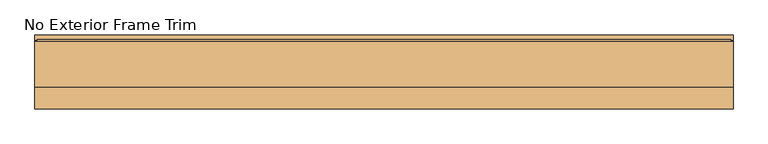
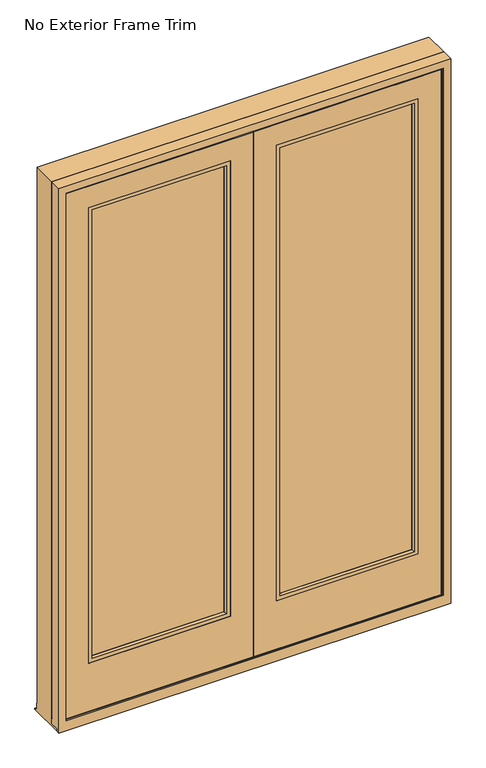
"""IFC4 building model written with IfcOpenShell, lengths in millimetres: door geometry, Door-In_Swing-Milgard-Essence-2_Panel : No Exterior Frame Trim."""

import ifcopenshell
import ifcopenshell.guid

model = None  # the IFC model being written
_history = None  # IfcOwnerHistory: only IFC2X3 demands one
_inside = {}  # id of a spatial element -> (the spatial element, [elements in it])
_under = {}  # id of a project, library or spatial element -> (it, [spatial elements below it])
_declared = {}  # id of a project -> (the project, [libraries it declares])
_typed = {}  # id of a type object -> (the type object, [elements of that type])
_made_of = {}  # id of a material, layer set ... -> (it, [elements and type objects made of it])


def new_model(schema):
    """Start an empty IFC model of exactly this schema.

    Asked for "IFC4X3", IfcOpenShell would pick the latest addendum, in which some entities
    have other attributes; the version numbers below select the first issue.
    IFC2X3 requires an IfcOwnerHistory on every rooted entity: one is made here for all.
    """
    global model, _history
    if schema == "IFC4X3":
        model = ifcopenshell.file(schema_version=(4, 3, 0, 0))
    else:
        model = ifcopenshell.file(schema=schema)
    _inside.clear()
    _under.clear()
    _declared.clear()
    _typed.clear()
    _made_of.clear()
    _history = None
    if model.schema == "IFC2X3":
        org = make("IfcOrganization", Name="unknown")
        user = make(
            "IfcPersonAndOrganization",
            ThePerson=make("IfcPerson", FamilyName="unknown"),
            TheOrganization=org,
        )
        app = make(
            "IfcApplication",
            ApplicationDeveloper=org,
            Version="unknown",
            ApplicationFullName="unknown",
            ApplicationIdentifier="unknown",
        )
        _history = make(
            "IfcOwnerHistory",
            OwningUser=user,
            OwningApplication=app,
            ChangeAction="ADDED",
            CreationDate=0,
        )
    return model


def make(cls, **values):
    """One entity of the class cls with the attributes given. An attribute that is None is left unset."""
    return model.create_entity(
        cls, **{name: value for name, value in values.items() if value is not None}
    )


def rooted(cls, **values):
    """An entity with a GlobalId (a new one), such as an element, a storey or a relation."""
    return make(cls, GlobalId=ifcopenshell.guid.new(), OwnerHistory=_history, **values)


def si_unit(unit_type, name, prefix=None):
    """IfcSIUnit, for example si_unit("LENGTHUNIT", "METRE", prefix="MILLI")."""
    return make("IfcSIUnit", UnitType=unit_type, Prefix=prefix, Name=name)


def assignment(units):
    """IfcUnitAssignment: the units of a project."""
    return None if units is None else make("IfcUnitAssignment", Units=units)


def point(xyz):
    """IfcCartesianPoint."""
    return None if xyz is None else make("IfcCartesianPoint", Coordinates=xyz)


def direction(xyz):
    """IfcDirection."""
    return None if xyz is None else make("IfcDirection", DirectionRatios=xyz)


def frame(location, z_axis=None, x_axis=None):
    """IfcAxis2Placement3D, a coordinate frame: its origin and axes. An axis left out is left unset."""
    return make(
        "IfcAxis2Placement3D",
        Location=point(location),
        Axis=direction(z_axis),
        RefDirection=direction(x_axis),
    )


def origin():
    """The frame at (0, 0, 0) with its axes left unset."""
    return frame((0.0, 0.0, 0.0))


def place(relative_to, where):
    """IfcLocalPlacement: puts the frame where relative to a parent placement (None: the world)."""
    return make(
        "IfcLocalPlacement", PlacementRelTo=relative_to, RelativePlacement=where
    )


def context(
    kind, dimensions, precision=None, world=None, true_north=None, identifier=None
):
    """IfcGeometricRepresentationContext, for example the 3D "Model" context."""
    return make(
        "IfcGeometricRepresentationContext",
        ContextIdentifier=identifier,
        ContextType=kind,
        CoordinateSpaceDimension=dimensions,
        Precision=precision,
        WorldCoordinateSystem=world,
        TrueNorth=true_north,
    )


def project(units=None, contexts=None):
    """IfcProject with its units and contexts."""
    return rooted(
        "IfcProject",
        Name="project",
        RepresentationContexts=contexts,
        UnitsInContext=assignment(units),
    )


def spatial(cls, under=None, at=None, **own):
    """A site, building, storey or space (cls), placed at a placement, below another one or the project."""
    s = rooted(cls, ObjectPlacement=at, **own)
    if under is not None:
        _under.setdefault(under.id(), (under, []))[1].append(s)
    return s


def polyline(points):
    """IfcPolyline through the points."""
    return make("IfcPolyline", Points=[point(p) for p in points])


def outline(outer, holes=None, kind="AREA"):
    """IfcArbitraryClosedProfileDef: a profile drawn as a closed curve; with holes, ...WithVoids."""
    if holes is None:
        return make("IfcArbitraryClosedProfileDef", ProfileType=kind, OuterCurve=outer)
    return make(
        "IfcArbitraryProfileDefWithVoids",
        ProfileType=kind,
        OuterCurve=outer,
        InnerCurves=holes,
    )


def extrude(swept, where, along, depth):
    """IfcExtrudedAreaSolid: the profile swept, set in the frame where, extruded along a direction by depth."""
    return make(
        "IfcExtrudedAreaSolid",
        SweptArea=swept,
        Position=where,
        ExtrudedDirection=direction(along),
        Depth=depth,
    )


def faces_of(points, faces, orient=None, outer=None):
    """IfcFace entities. A face is a list of loops; a loop is a list of indices into points, from 0.

    orient and outer hold one flag for each loop. By default every Orientation is true, the
    first loop of a face is its IfcFaceOuterBound and the others are IfcFaceBound.
    """
    made = []
    for i, loops in enumerate(faces):
        bounds = []
        for j, loop in enumerate(loops):
            is_outer = j == 0 if outer is None else outer[i][j]
            bounds.append(
                make(
                    "IfcFaceOuterBound" if is_outer else "IfcFaceBound",
                    Bound=make("IfcPolyLoop", Polygon=[points[k] for k in loop]),
                    Orientation=True if orient is None else orient[i][j],
                )
            )
        made.append(make("IfcFace", Bounds=bounds))
    return made


def faceted_brep(points, faces, orient=None, outer=None, voids=None):
    """IfcFacetedBrep: a solid bounded by flat faces; with voids (closed shells), ...WithVoids."""
    shared = [point(p) for p in points]
    hull = make("IfcClosedShell", CfsFaces=faces_of(shared, faces, orient, outer))
    if voids is None:
        return make("IfcFacetedBrep", Outer=hull)
    return make(
        "IfcFacetedBrepWithVoids",
        Outer=hull,
        Voids=[
            make(cls, CfsFaces=faces_of(shared, fs, o, b)) for cls, fs, o, b in voids
        ],
    )


def shape(context_of_items, identifier, shape_type, items):
    """IfcShapeRepresentation: the items that make up one representation, for example the "Body"."""
    return make(
        "IfcShapeRepresentation",
        ContextOfItems=context_of_items,
        RepresentationIdentifier=identifier,
        RepresentationType=shape_type,
        Items=items,
    )


def source(mapping_origin, context_of_items, identifier, shape_type, items):
    """IfcRepresentationMap: a shape defined once, which mapped items show again and again."""
    return make(
        "IfcRepresentationMap",
        MappingOrigin=mapping_origin,
        MappedRepresentation=shape(context_of_items, identifier, shape_type, items),
    )


def transform(
    local_origin,
    x_axis=None,
    y_axis=None,
    z_axis=None,
    scale=None,
    scale2=None,
    scale3=None,
    uniform=True,
):
    """IfcCartesianTransformationOperator3D, or its non-uniform kind. x_axis, y_axis, z_axis: its Axis1, 2, 3."""
    if uniform:
        return make(
            "IfcCartesianTransformationOperator3D",
            Axis1=direction(x_axis),
            Axis2=direction(y_axis),
            LocalOrigin=point(local_origin),
            Scale=scale,
            Axis3=direction(z_axis),
        )
    return make(
        "IfcCartesianTransformationOperator3DnonUniform",
        Axis1=direction(x_axis),
        Axis2=direction(y_axis),
        LocalOrigin=point(local_origin),
        Scale=scale,
        Axis3=direction(z_axis),
        Scale2=scale2,
        Scale3=scale3,
    )


def mapped(mapping_source, mapping_target):
    """IfcMappedItem: shows the shape of a source again, moved by a transform."""
    return make(
        "IfcMappedItem", MappingSource=mapping_source, MappingTarget=mapping_target
    )


def made_of(thing, what):
    """Note that an element or type object is made of a material, layer set ...; save() writes the relation."""
    if what is not None:
        _made_of.setdefault(what.id(), (what, []))[1].append(thing)
    return thing


def element(
    cls,
    number,
    at=None,
    inside=None,
    cuts=None,
    type_object=None,
    material=None,
    context=None,
    identifier="Body",
    shape_type=None,
    held_by="IfcProductDefinitionShape",
    body=None,
    shapes=None,
    **own,
):
    """One element of the class cls, such as IfcWall. Its Tag is "e" and its number.

    at: its placement. inside: the storey or other place that contains it. cuts: it is an
    opening in that element (IfcRelVoidsElement). A single representation is given by context,
    identifier, shape_type and body (its items); several are given by shapes. held_by: the class
    of the entity that holds the representations. save() writes the other relations.
    """
    e = rooted(cls, Tag="e%d" % number, ObjectPlacement=at, **own)
    if body is not None:
        shapes = [shape(context, identifier, shape_type, body)]
    if shapes is not None:
        e.Representation = make(held_by, Representations=shapes)
    if inside is not None:
        _inside.setdefault(inside.id(), (inside, []))[1].append(e)
    if cuts is not None:
        rooted(
            "IfcRelVoidsElement", RelatingBuildingElement=cuts, RelatedOpeningElement=e
        )
    if type_object is not None:
        _typed.setdefault(type_object.id(), (type_object, []))[1].append(e)
    return made_of(e, material)


def aggregate(whole, parts):
    """IfcRelAggregates: a whole, such as a stair, and the parts it consists of."""
    return rooted("IfcRelAggregates", RelatingObject=whole, RelatedObjects=parts)


def save(model, path):
    """Write the relations noted so far, then the file.

    IfcRelAggregates (storeys below a building ...), IfcRelContainedInSpatialStructure (elements
    in a storey), IfcRelDefinesByType, IfcRelAssociatesMaterial and IfcRelDeclares: one each for
    every whole, place, type object, material and project.
    """
    for whole, parts in _under.values():
        aggregate(whole, parts)
    for where, things in _inside.values():
        rooted(
            "IfcRelContainedInSpatialStructure",
            RelatedElements=things,
            RelatingStructure=where,
        )
    for kind, things in _typed.values():
        rooted("IfcRelDefinesByType", RelatedObjects=things, RelatingType=kind)
    for what, things in _made_of.values():
        rooted("IfcRelAssociatesMaterial", RelatedObjects=things, RelatingMaterial=what)
    for by, libraries in _declared.values():
        rooted("IfcRelDeclares", RelatingContext=by, RelatedDefinitions=libraries)
    model.write(path)


def no_exterior_frame_trim_3783c24b(model_context):
    return source(origin(), model_context, "Body", "SolidModel", [
        extrude(outline(polyline([(591.4684989, -28.575), (591.4684989, -53.975), (54.2422052, -53.975), (54.2422052, -28.575), (591.4684989, -28.575)])), frame((0.0, 0.0, 245.0465023), z_axis=(0.0, 0.0, 1.0), x_axis=(1.0, 0.0, 0.0)), (0.0, 0.0, 1.0), 1856.965426),
        faceted_brep([(-22.501829, -56.3244996, 39.0524923), (-20.0336081, -53.2765006, 39.0524923), (47.7525111, -53.2765006, 39.0524923), (47.7525111, -55.0418002, 39.0524923), (61.9460004, -55.0418002, 39.0524923), (63.4695489, -53.975, 39.0524923), (66.9526032, -53.975, 39.0524923), (66.9526032, -55.857139, 39.0524923), (66.6827722, -56.3244996, 39.0524923), (579.0279319, -56.3244996, 39.0524923), (578.7581009, -55.857139, 39.0524923), (578.7581009, -53.975, 39.0524923), (582.2411552, -53.975, 39.0524923), (583.7647037, -55.0418002, 39.0524923), (597.9581931, -55.0418002, 39.0524923), (597.9581931, -53.2765006, 39.0524923), (665.7443122, -53.2765006, 39.0524923), (668.2125331, -56.3244996, 39.0524923), (685.524688, -56.3244996, 39.0524923), (685.524688, -64.6430002, 39.0524923), (-39.8139839, -64.6430002, 39.0524923), (-39.8139839, -56.3244996, 39.0524923), (-22.501829, -56.3244996, 56.3603664), (-20.0336081, -53.2765006, 58.8285873), (-22.501829, -56.3244996, 2178.7559624), (-20.0336081, -53.2765006, 2176.2877415), (-20.0336081, -53.2765006, 238.4932696), (-21.4631194, -55.0418002, 238.4932696), (-21.4631194, -55.0418002, 252.686759), (-20.5992417, -53.975, 254.2103075), (-20.5992417, -53.975, 257.6933617), (-22.1233678, -55.857139, 257.6933617), (-22.501829, -56.3244996, 257.4235308), (-39.8139839, -53.2765006, 58.8285873), (-39.8139839, -53.2765006, 238.4932696), (665.7443122, -53.2765006, 2176.2877415), (665.7443122, -53.2765006, 238.4932696), (685.524688, -53.2765006, 238.4932696), (685.524688, -53.2765006, 58.8285873), (665.7443122, -53.2765006, 58.8285873), (597.9581931, -53.2765006, 58.8285873), (47.7525111, -53.2765006, 58.8285873), (47.7525111, -53.2765006, 2108.5016224), (47.7525111, -53.2765006, 238.4932696), (597.9581931, -53.2765006, 238.4932696), (597.9581931, -53.2765006, 2108.5016224), (47.7525111, -55.0418002, 57.3990759), (47.7525111, -55.0418002, 2108.5016224), (47.7525111, -55.0418002, 257.6933617), (47.7525111, -53.975, 257.6933617), (47.7525111, -53.975, 254.2103075), (47.7525111, -55.0418002, 252.686759), (47.7525111, -55.0418002, 238.4932696), (61.9460004, -55.0418002, 57.3990759), (583.7647037, -55.0418002, 57.3990759), (597.9581931, -55.0418002, 57.3990759), (61.9460004, -55.0418002, 252.686759), (61.9460004, -55.0418002, 238.4932696), (597.9581931, -55.0418002, 2108.5016224), (597.9581931, -55.0418002, 257.6933617), (583.7647037, -55.0418002, 257.6933617), (583.7647037, -55.0418002, 2094.3081331), (61.9460004, -55.0418002, 2094.3081331), (61.9460004, -55.0418002, 257.6933617), (597.9581931, -55.0418002, 252.686759), (597.9581931, -55.0418002, 238.4932696), (583.7647037, -55.0418002, 238.4932696), (583.7647037, -55.0418002, 252.686759), (63.4695489, -53.975, 58.2629537), (63.4695489, -53.975, 254.2103075), (63.4695489, -53.975, 238.4932696), (63.4695489, -53.975, 2092.7845845), (63.4695489, -53.975, 257.6933617), (66.9526032, -53.975, 58.2629537), (578.7581009, -53.975, 58.2629537), (582.2411552, -53.975, 58.2629537), (582.2411552, -53.975, 2092.7845845), (582.2411552, -53.975, 257.6933617), (597.9581931, -53.975, 257.6933617), (597.9581931, -53.975, 254.2103075), (582.2411552, -53.975, 254.2103075), (582.2411552, -53.975, 238.4932696), (578.7581009, -53.975, 238.4932696), (578.7581009, -53.975, 254.2103075), (66.9526032, -53.975, 254.2103075), (66.9526032, -53.975, 238.4932696), (66.9526032, -53.975, 2089.3015303), (66.9526032, -53.975, 257.6933617), (578.7581009, -53.975, 257.6933617), (578.7581009, -53.975, 2089.3015303), (-39.8139839, -53.975, 254.2103075), (-39.8139839, -53.975, 257.6933617), (685.524688, -53.975, 257.6933617), (685.524688, -53.975, 254.2103075), (666.3099458, -53.975, 254.2103075), (666.3099458, -53.975, 257.6933617), (66.9526032, -55.857139, 56.7388275), (66.9526032, -55.0418002, 252.686759), (66.9526032, -55.0418002, 238.4932696), (66.9526032, -55.857139, 2089.3015303), (66.9526032, -55.857139, 257.6933617), (66.6827722, -56.3244996, 56.3603664), (62.3383529, -63.8492502, 2093.9157805), (62.3383529, -63.8492502, 253.0791115), (597.9581931, -63.8492502, 2108.5016224), (47.7525111, -63.8492502, 2108.5016224), (47.7525111, -63.8492502, 238.4932696), (597.9581931, -63.8492502, 238.4932696), (583.3723512, -63.8492502, 2093.9157805), (583.3723512, -63.8492502, 253.0791115), (47.7525111, -64.6430002, 2108.5016224), (47.7525111, -64.6430002, 238.4932696), (685.524688, -64.6430002, 2196.0681173), (-39.8139839, -64.6430002, 2196.0681173), (597.9581931, -64.6430002, 2108.5016224), (597.9581931, -64.6430002, 238.4932696), (-39.8139839, -56.3244996, 2196.0681173), (-39.8139839, -56.3244996, 257.4235308), (-39.8139839, -55.857139, 257.6933617), (-39.8139839, -55.0418002, 252.686759), (-39.8139839, -55.0418002, 238.4932696), (-39.8139839, -56.3244996, 56.3603664), (668.2125331, -56.3244996, 56.3603664), (685.524688, -56.3244996, 56.3603664), (685.524688, -56.3244996, 2196.0681173), (685.524688, -56.3244996, 257.4235308), (668.2125331, -56.3244996, 257.4235308), (668.2125331, -56.3244996, 2178.7559624), (578.7581009, -55.857139, 2089.3015303), (667.8340719, -55.857139, 257.6933617), (667.1738236, -55.0418002, 252.686759), (667.1738236, -55.0418002, 238.4932696), (578.7581009, -55.857139, 56.7388275), (578.7581009, -55.857139, 257.6933617), (578.7581009, -55.0418002, 238.4932696), (578.7581009, -55.0418002, 252.686759), (579.0279319, -56.3244996, 56.3603664), (685.524688, -55.0418002, 238.4932696), (685.524688, -55.0418002, 252.686759), (685.524688, -55.857139, 257.6933617)], [[[0, 1, 2, 3, 4, 5, 6, 7, 8, 9, 10, 11, 12, 13, 14, 15, 16, 17, 18, 19, 20, 21]], [[1, 0, 22, 23]], [[24, 25, 26, 27, 28, 29, 30, 31, 32]], [[2, 1, 23, 33, 34, 26, 25, 35, 36, 37, 38, 39, 16, 15, 40, 41], [42, 43, 44, 45]], [[3, 2, 41, 46]], [[42, 47, 48, 49, 50, 51, 52, 43]], [[4, 3, 46, 53]], [[14, 13, 54, 55]], [[52, 51, 56, 57]], [[47, 58, 59, 60, 61, 62, 63, 48]], [[64, 65, 66, 67]], [[5, 4, 53, 68]], [[57, 56, 69, 70]], [[62, 71, 72, 63]], [[6, 5, 68, 73]], [[12, 11, 74, 75]], [[71, 76, 77, 78, 79, 80, 81, 82, 83, 84, 85, 70, 69, 50, 49, 72], [86, 87, 88, 89]], [[90, 91, 30, 29]], [[92, 93, 94, 95]], [[7, 6, 73, 96]], [[85, 84, 97, 98]], [[86, 99, 100, 87]], [[8, 7, 96, 101]], [[99, 102, 103, 100]], [[104, 105, 106, 107], [102, 108, 109, 103]], [[106, 105, 110, 111]], [[20, 19, 112, 113], [114, 115, 111, 110]], [[21, 20, 113, 116, 117, 118, 91, 90, 119, 120, 34, 33, 121]], [[18, 17, 122, 123]], [[0, 21, 121, 22]], [[116, 124, 125, 126, 127, 24, 32, 117]], [[25, 24, 127, 35]], [[42, 45, 58, 47]], [[62, 61, 76, 71]], [[86, 89, 128, 99]], [[102, 99, 128, 108]], [[105, 104, 114, 110]], [[113, 112, 124, 116]], [[17, 16, 39, 122]], [[35, 127, 126, 129, 95, 94, 130, 131, 36]], [[15, 14, 55, 40]], [[58, 45, 44, 65, 64, 79, 78, 59]], [[13, 12, 75, 54]], [[81, 80, 67, 66]], [[76, 61, 60, 77]], [[11, 10, 132, 74]], [[128, 89, 88, 133]], [[83, 82, 134, 135]], [[10, 9, 136, 132]], [[108, 128, 133, 109]], [[114, 104, 107, 115]], [[124, 112, 19, 18, 123, 38, 37, 137, 138, 93, 92, 139, 125]], [[107, 106, 111, 115]], [[118, 117, 32, 31]], [[125, 139, 129, 126]], [[103, 109, 133, 100]], [[78, 77, 60, 59]], [[72, 49, 48, 63]], [[88, 87, 100, 133]], [[91, 118, 31, 30]], [[139, 92, 95, 129]], [[119, 90, 29, 28]], [[93, 138, 130, 94]], [[80, 79, 64, 67]], [[84, 83, 135, 97]], [[50, 69, 56, 51]], [[120, 119, 28, 27]], [[138, 137, 131, 130]], [[97, 135, 134, 98]], [[44, 43, 52, 57, 70, 85, 98, 134, 82, 81, 66, 65]], [[34, 120, 27, 26]], [[137, 37, 36, 131]], [[121, 33, 23, 22]], [[38, 123, 122, 39]], [[41, 40, 55, 54, 75, 74, 132, 136, 101, 96, 73, 68, 53, 46]], [[9, 8, 101, 136]]]),
        faceted_brep([(-39.8139839, -20.1929984, 39.0524923), (-39.8139839, -56.3244996, 39.0524923), (-39.8139839, -56.3244996, 2196.0681173), (-39.8139839, -20.1929984, 2196.0681173), (685.524688, -56.3244996, 39.0524923), (685.524688, -20.1929984, 39.0524923), (685.524688, -20.1929984, 2196.0681173), (685.524688, -56.3244996, 2196.0681173), (66.7863819, -27.3270033, 257.5271404), (578.9243222, -27.3270033, 257.5271404), (586.0583272, -20.1929984, 250.3931355), (59.6523769, -20.1929984, 250.3931355), (586.0583272, -20.1929984, 2096.6017565), (59.6523769, -20.1929984, 2096.6017565), (669.6356705, -56.3244996, 55.4786786), (-23.9249664, -56.3244996, 55.4786786), (-23.9249664, -56.3244996, 2180.1790999), (669.6356705, -56.3244996, 2180.1790999), (666.5876715, -53.2765006, 57.9468995), (-20.8769674, -53.2765006, 57.9468995), (666.5876715, -53.2765006, 2177.1311009), (-20.8769674, -53.2765006, 2177.1311009), (594.7531877, -53.2765006, 241.698275), (50.9575164, -53.2765006, 241.698275), (50.9575164, -53.2765006, 2105.296617), (594.7531877, -53.2765006, 2105.296617), (594.7531877, -50.8481081, 241.698275), (50.9575164, -50.8481081, 241.698275), (49.0643221, -50.8481081, 2107.1898114), (596.646382, -50.8481081, 2107.1898114), (596.646382, -50.8481081, 239.8050807), (49.0643221, -50.8481081, 239.8050807), (594.7531877, -50.8481081, 2105.296617), (50.9575164, -50.8481081, 2105.296617), (597.9581931, -46.8107689, 238.4932696), (47.7525111, -46.8107689, 238.4932696), (597.9581931, -27.8384005, 238.4932696), (581.6983611, -27.8384005, 238.4932696), (580.9617616, -28.575, 238.4932696), (578.9243222, -28.575, 238.4932696), (578.9243222, -27.8384005, 238.4932696), (66.7863819, -27.8384005, 238.4932696), (66.7863819, -28.575, 238.4932696), (64.7489425, -28.575, 238.4932696), (64.012343, -27.8384005, 238.4932696), (47.7525111, -27.8384005, 238.4932696), (597.9581931, -27.8384005, 254.7531016), (581.6983611, -27.8384005, 254.7531016), (578.9243222, -27.8384005, 254.7531016), (66.7863819, -27.8384005, 254.7531016), (64.012343, -27.8384005, 254.7531016), (47.7525111, -27.8384005, 254.7531016), (64.7489425, -28.575, 255.4897011), (47.7525111, -28.575, 255.4897011), (578.9243222, -28.575, 255.4897011), (66.7863819, -28.575, 255.4897011), (597.9581931, -28.575, 255.4897011), (580.9617616, -28.575, 255.4897011), (597.9581931, -28.575, 257.5271404), (580.9617616, -28.575, 257.5271404), (580.9617616, -28.575, 2091.505191), (64.7489425, -28.575, 2091.505191), (64.7489425, -28.575, 257.5271404), (47.7525111, -28.575, 257.5271404), (578.9243222, -28.575, 257.5271404), (66.7863819, -28.575, 257.5271404), (66.7863819, -28.575, 2089.4677516), (578.9243222, -28.575, 2089.4677516), (597.9581931, -27.8384005, 257.5271404), (581.6983611, -27.8384005, 257.5271404), (64.012343, -27.8384005, 257.5271404), (47.7525111, -27.8384005, 257.5271404), (66.7863819, -27.3270033, 2089.4677516), (64.012343, -27.8384005, 2092.2417904), (581.6983611, -27.8384005, 2092.2417904), (597.9581931, -27.8384005, 2108.5016224), (47.7525111, -27.8384005, 2108.5016224), (47.7525111, -46.8107689, 2108.5016224), (578.9243222, -27.3270033, 2089.4677516), (597.9581931, -46.8107689, 2108.5016224)], [[[0, 1, 2, 3]], [[4, 5, 6, 7]], [[8, 9, 10, 11]], [[0, 3, 6, 5], [11, 10, 12, 13]], [[4, 1, 0, 5]], [[2, 1, 4, 7], [14, 15, 16, 17]], [[15, 14, 18, 19]], [[20, 21, 19, 18], [22, 23, 24, 25]], [[23, 22, 26, 27]], [[28, 29, 30, 31], [27, 26, 32, 33]], [[31, 30, 34, 35]], [[35, 34, 36, 37, 38, 39, 40, 41, 42, 43, 44, 45]], [[37, 36, 46, 47]], [[41, 40, 48, 49]], [[45, 44, 50, 51]], [[51, 50, 52, 53]], [[49, 48, 54, 55]], [[47, 46, 56, 57]], [[53, 52, 43, 42, 55, 54, 39, 38, 57, 56, 58, 59, 60, 61, 62, 63], [64, 65, 66, 67]], [[9, 8, 65, 64]], [[59, 58, 68, 69]], [[63, 62, 70, 71]], [[13, 72, 8, 11]], [[55, 42, 41, 49]], [[72, 66, 65, 8]], [[43, 52, 50, 44]], [[61, 73, 70, 62]], [[73, 74, 69, 68, 75, 76, 71, 70]], [[76, 77, 35, 45, 51, 53, 63, 71]], [[77, 28, 31, 35]], [[33, 24, 23, 27]], [[19, 21, 16, 15]], [[13, 12, 78, 72]], [[66, 72, 78, 67]], [[61, 60, 74, 73]], [[76, 75, 79, 77]], [[28, 77, 79, 29]], [[33, 32, 25, 24]], [[21, 20, 17, 16]], [[6, 3, 2, 7]], [[78, 12, 10, 9]], [[39, 54, 48, 40]], [[67, 78, 9, 64]], [[74, 60, 59, 69]], [[57, 38, 37, 47]], [[79, 75, 68, 58, 56, 46, 36, 34]], [[30, 29, 79, 34]], [[25, 32, 26, 22]], [[17, 20, 18, 14]]]),
        extrude(outline(polyline([(-675.754549, -28.575), (-138.5282552, -28.575), (-138.5282552, -53.975), (-675.754549, -53.975), (-675.754549, -28.575)])), frame((0.0, 0.0, 245.0465023), z_axis=(0.0, 0.0, 1.0), x_axis=(1.0, 0.0, 0.0)), (0.0, 0.0, 1.0), 1856.965426),
        faceted_brep([(-61.784221, -56.3244996, 39.0524923), (-44.4720661, -56.3244996, 39.0524923), (-44.4720661, -64.6430002, 39.0524923), (-769.810738, -64.6430002, 39.0524923), (-769.810738, -56.3244996, 39.0524923), (-752.4985831, -56.3244996, 39.0524923), (-750.0303622, -53.2765006, 39.0524923), (-682.2442431, -53.2765006, 39.0524923), (-682.2442431, -55.0418002, 39.0524923), (-668.0507537, -55.0418002, 39.0524923), (-666.5272052, -53.975, 39.0524923), (-663.044151, -53.975, 39.0524923), (-663.044151, -55.857139, 39.0524923), (-663.3139819, -56.3244996, 39.0524923), (-150.9688223, -56.3244996, 39.0524923), (-151.2386532, -55.857139, 39.0524923), (-151.2386532, -53.975, 39.0524923), (-147.755599, -53.975, 39.0524923), (-146.2320504, -55.0418002, 39.0524923), (-132.0385611, -55.0418002, 39.0524923), (-132.0385611, -53.2765006, 39.0524923), (-64.252442, -53.2765006, 39.0524923), (-61.784221, -56.3244996, 2178.7559624), (-61.784221, -56.3244996, 257.4235308), (-62.1626822, -55.857139, 257.6933617), (-63.6868083, -53.975, 257.6933617), (-63.6868083, -53.975, 254.2103075), (-62.8229306, -55.0418002, 252.686759), (-62.8229306, -55.0418002, 238.4932696), (-64.252442, -53.2765006, 238.4932696), (-64.252442, -53.2765006, 2176.2877415), (-64.252442, -53.2765006, 58.8285873), (-61.784221, -56.3244996, 56.3603664), (-132.0385611, -53.2765006, 58.8285873), (-682.2442431, -53.2765006, 58.8285873), (-750.0303622, -53.2765006, 58.8285873), (-769.810738, -53.2765006, 58.8285873), (-769.810738, -53.2765006, 238.4932696), (-750.0303622, -53.2765006, 238.4932696), (-750.0303622, -53.2765006, 2176.2877415), (-44.4720661, -53.2765006, 238.4932696), (-44.4720661, -53.2765006, 58.8285873), (-132.0385611, -53.2765006, 2108.5016224), (-682.2442431, -53.2765006, 2108.5016224), (-682.2442431, -53.2765006, 238.4932696), (-132.0385611, -53.2765006, 238.4932696), (-132.0385611, -55.0418002, 238.4932696), (-132.0385611, -55.0418002, 252.686759), (-132.0385611, -53.975, 254.2103075), (-132.0385611, -53.975, 257.6933617), (-132.0385611, -55.0418002, 257.6933617), (-132.0385611, -55.0418002, 2108.5016224), (-132.0385611, -55.0418002, 57.3990759), (-146.2320504, -55.0418002, 257.6933617), (-146.2320504, -55.0418002, 2094.3081331), (-668.0507537, -55.0418002, 2094.3081331), (-668.0507537, -55.0418002, 257.6933617), (-682.2442431, -55.0418002, 257.6933617), (-682.2442431, -55.0418002, 2108.5016224), (-682.2442431, -55.0418002, 57.3990759), (-668.0507537, -55.0418002, 57.3990759), (-146.2320504, -55.0418002, 238.4932696), (-146.2320504, -55.0418002, 252.686759), (-682.2442431, -55.0418002, 252.686759), (-668.0507537, -55.0418002, 252.686759), (-668.0507537, -55.0418002, 238.4932696), (-682.2442431, -55.0418002, 238.4932696), (-146.2320504, -55.0418002, 57.3990759), (-147.755599, -53.975, 257.6933617), (-147.755599, -53.975, 2092.7845845), (-147.755599, -53.975, 238.4932696), (-147.755599, -53.975, 254.2103075), (-147.755599, -53.975, 58.2629537), (-151.2386532, -53.975, 238.4932696), (-151.2386532, -53.975, 254.2103075), (-663.044151, -53.975, 254.2103075), (-663.044151, -53.975, 238.4932696), (-666.5272052, -53.975, 238.4932696), (-666.5272052, -53.975, 254.2103075), (-682.2442431, -53.975, 254.2103075), (-682.2442431, -53.975, 257.6933617), (-666.5272052, -53.975, 257.6933617), (-666.5272052, -53.975, 2092.7845845), (-151.2386532, -53.975, 2089.3015303), (-663.044151, -53.975, 2089.3015303), (-663.044151, -53.975, 257.6933617), (-151.2386532, -53.975, 257.6933617), (-666.5272052, -53.975, 58.2629537), (-663.044151, -53.975, 58.2629537), (-769.810738, -53.975, 257.6933617), (-750.5959958, -53.975, 257.6933617), (-750.5959958, -53.975, 254.2103075), (-769.810738, -53.975, 254.2103075), (-151.2386532, -53.975, 58.2629537), (-44.4720661, -53.975, 254.2103075), (-44.4720661, -53.975, 257.6933617), (-151.2386532, -55.857139, 257.6933617), (-151.2386532, -55.857139, 2089.3015303), (-151.2386532, -55.0418002, 238.4932696), (-151.2386532, -55.0418002, 252.686759), (-151.2386532, -55.857139, 56.7388275), (-146.624403, -63.8492502, 253.0791115), (-146.624403, -63.8492502, 2093.9157805), (-150.9688223, -56.3244996, 56.3603664), (-682.2442431, -63.8492502, 2108.5016224), (-682.2442431, -63.8492502, 238.4932696), (-132.0385611, -63.8492502, 238.4932696), (-132.0385611, -63.8492502, 2108.5016224), (-667.6584012, -63.8492502, 253.0791115), (-667.6584012, -63.8492502, 2093.9157805), (-132.0385611, -64.6430002, 238.4932696), (-132.0385611, -64.6430002, 2108.5016224), (-44.4720661, -64.6430002, 2196.0681173), (-769.810738, -64.6430002, 2196.0681173), (-682.2442431, -64.6430002, 2108.5016224), (-682.2442431, -64.6430002, 238.4932696), (-44.4720661, -56.3244996, 56.3603664), (-44.4720661, -55.0418002, 238.4932696), (-44.4720661, -55.0418002, 252.686759), (-44.4720661, -55.857139, 257.6933617), (-44.4720661, -56.3244996, 257.4235308), (-44.4720661, -56.3244996, 2196.0681173), (-752.4985831, -56.3244996, 2178.7559624), (-752.4985831, -56.3244996, 257.4235308), (-769.810738, -56.3244996, 257.4235308), (-769.810738, -56.3244996, 2196.0681173), (-769.810738, -56.3244996, 56.3603664), (-752.4985831, -56.3244996, 56.3603664), (-663.044151, -55.857139, 2089.3015303), (-751.4598736, -55.0418002, 238.4932696), (-751.4598736, -55.0418002, 252.686759), (-752.120122, -55.857139, 257.6933617), (-663.044151, -55.857139, 56.7388275), (-663.044151, -55.0418002, 252.686759), (-663.044151, -55.0418002, 238.4932696), (-663.044151, -55.857139, 257.6933617), (-663.3139819, -56.3244996, 56.3603664), (-769.810738, -55.857139, 257.6933617), (-769.810738, -55.0418002, 252.686759), (-769.810738, -55.0418002, 238.4932696)], [[[0, 1, 2, 3, 4, 5, 6, 7, 8, 9, 10, 11, 12, 13, 14, 15, 16, 17, 18, 19, 20, 21]], [[22, 23, 24, 25, 26, 27, 28, 29, 30]], [[21, 31, 32, 0]], [[20, 33, 34, 7, 6, 35, 36, 37, 38, 39, 30, 29, 40, 41, 31, 21], [42, 43, 44, 45]], [[42, 45, 46, 47, 48, 49, 50, 51]], [[19, 52, 33, 20]], [[51, 50, 53, 54, 55, 56, 57, 58]], [[8, 59, 60, 9]], [[46, 61, 62, 47]], [[63, 64, 65, 66]], [[18, 67, 52, 19]], [[54, 53, 68, 69]], [[61, 70, 71, 62]], [[17, 72, 67, 18]], [[69, 68, 49, 48, 71, 70, 73, 74, 75, 76, 77, 78, 79, 80, 81, 82], [83, 84, 85, 86]], [[10, 87, 88, 11]], [[89, 90, 91, 92]], [[16, 93, 72, 17]], [[94, 26, 25, 95]], [[83, 86, 96, 97]], [[73, 98, 99, 74]], [[15, 100, 93, 16]], [[97, 96, 101, 102]], [[14, 103, 100, 15]], [[104, 105, 106, 107], [102, 101, 108, 109]], [[106, 110, 111, 107]], [[2, 112, 113, 3], [114, 111, 110, 115]], [[1, 116, 41, 40, 117, 118, 94, 95, 119, 120, 121, 112, 2]], [[0, 32, 116, 1]], [[121, 120, 23, 22, 122, 123, 124, 125]], [[4, 126, 127, 5]], [[30, 39, 122, 22]], [[42, 51, 58, 43]], [[54, 69, 82, 55]], [[83, 97, 128, 84]], [[102, 109, 128, 97]], [[107, 111, 114, 104]], [[112, 121, 125, 113]], [[39, 38, 129, 130, 91, 90, 131, 123, 122]], [[5, 127, 35, 6]], [[58, 57, 80, 79, 63, 66, 44, 43]], [[7, 34, 59, 8]], [[82, 81, 56, 55]], [[9, 60, 87, 10]], [[77, 65, 64, 78]], [[11, 88, 132, 12]], [[75, 133, 134, 76]], [[128, 135, 85, 84]], [[109, 108, 135, 128]], [[12, 132, 136, 13]], [[114, 115, 105, 104]], [[125, 124, 137, 89, 92, 138, 139, 37, 36, 126, 4, 3, 113]], [[105, 115, 110, 106]], [[101, 96, 135, 108]], [[124, 123, 131, 137]], [[119, 24, 23, 120]], [[68, 53, 50, 49]], [[95, 25, 24, 119]], [[80, 57, 56, 81]], [[85, 135, 96, 86]], [[137, 131, 90, 89]], [[48, 47, 62, 71]], [[74, 99, 133, 75]], [[78, 64, 63, 79]], [[92, 91, 130, 138]], [[118, 27, 26, 94]], [[99, 98, 134, 133]], [[138, 130, 129, 139]], [[117, 28, 27, 118]], [[40, 29, 28, 117]], [[44, 66, 65, 77, 76, 134, 98, 73, 70, 61, 46, 45]], [[139, 129, 38, 37]], [[33, 52, 67, 72, 93, 100, 103, 136, 132, 88, 87, 60, 59, 34]], [[116, 32, 31, 41]], [[36, 35, 127, 126]], [[13, 136, 103, 14]]]),
        faceted_brep([(-44.4720661, -20.1929984, 39.0524923), (-44.4720661, -20.1929984, 2196.0681173), (-44.4720661, -56.3244996, 2196.0681173), (-44.4720661, -56.3244996, 39.0524923), (-769.810738, -56.3244996, 39.0524923), (-769.810738, -56.3244996, 2196.0681173), (-769.810738, -20.1929984, 2196.0681173), (-769.810738, -20.1929984, 39.0524923), (-151.0724319, -27.3270033, 257.5271404), (-143.938427, -20.1929984, 250.3931355), (-670.3443772, -20.1929984, 250.3931355), (-663.2103723, -27.3270033, 257.5271404), (-143.938427, -20.1929984, 2096.6017565), (-670.3443772, -20.1929984, 2096.6017565), (-753.9217206, -56.3244996, 55.4786786), (-753.9217206, -56.3244996, 2180.1790999), (-60.3610836, -56.3244996, 2180.1790999), (-60.3610836, -56.3244996, 55.4786786), (-63.4090826, -53.2765006, 57.9468995), (-750.8737216, -53.2765006, 57.9468995), (-750.8737216, -53.2765006, 2177.1311009), (-63.4090826, -53.2765006, 2177.1311009), (-679.0392377, -53.2765006, 241.698275), (-679.0392377, -53.2765006, 2105.296617), (-135.2435664, -53.2765006, 2105.296617), (-135.2435664, -53.2765006, 241.698275), (-135.2435664, -50.8481081, 241.698275), (-679.0392377, -50.8481081, 241.698275), (-133.3503721, -50.8481081, 2107.1898114), (-133.3503721, -50.8481081, 239.8050807), (-680.9324321, -50.8481081, 239.8050807), (-680.9324321, -50.8481081, 2107.1898114), (-135.2435664, -50.8481081, 2105.296617), (-679.0392377, -50.8481081, 2105.296617), (-132.0385611, -46.8107689, 238.4932696), (-682.2442431, -46.8107689, 238.4932696), (-132.0385611, -27.8384005, 238.4932696), (-148.298393, -27.8384005, 238.4932696), (-149.0349925, -28.575, 238.4932696), (-151.0724319, -28.575, 238.4932696), (-151.0724319, -27.8384005, 238.4932696), (-663.2103723, -27.8384005, 238.4932696), (-663.2103723, -28.575, 238.4932696), (-665.2478116, -28.575, 238.4932696), (-665.9844111, -27.8384005, 238.4932696), (-682.2442431, -27.8384005, 238.4932696), (-132.0385611, -27.8384005, 254.7531016), (-148.298393, -27.8384005, 254.7531016), (-151.0724319, -27.8384005, 254.7531016), (-663.2103723, -27.8384005, 254.7531016), (-665.9844111, -27.8384005, 254.7531016), (-682.2442431, -27.8384005, 254.7531016), (-132.0385611, -28.575, 255.4897011), (-149.0349925, -28.575, 255.4897011), (-151.0724319, -28.575, 255.4897011), (-663.2103723, -28.575, 255.4897011), (-665.2478116, -28.575, 255.4897011), (-682.2442431, -28.575, 255.4897011), (-132.0385611, -28.575, 257.5271404), (-149.0349925, -28.575, 257.5271404), (-149.0349925, -28.575, 2091.505191), (-665.2478116, -28.575, 2091.505191), (-665.2478116, -28.575, 257.5271404), (-682.2442431, -28.575, 257.5271404), (-663.2103723, -28.575, 257.5271404), (-663.2103723, -28.575, 2089.4677516), (-151.0724319, -28.575, 2089.4677516), (-151.0724319, -28.575, 257.5271404), (-132.0385611, -27.8384005, 257.5271404), (-148.298393, -27.8384005, 257.5271404), (-665.9844111, -27.8384005, 257.5271404), (-682.2442431, -27.8384005, 257.5271404), (-151.0724319, -27.3270033, 2089.4677516), (-148.298393, -27.8384005, 2092.2417904), (-132.0385611, -27.8384005, 2108.5016224), (-682.2442431, -27.8384005, 2108.5016224), (-665.9844111, -27.8384005, 2092.2417904), (-132.0385611, -46.8107689, 2108.5016224), (-663.2103723, -27.3270033, 2089.4677516), (-682.2442431, -46.8107689, 2108.5016224)], [[[0, 1, 2, 3]], [[4, 5, 6, 7]], [[8, 9, 10, 11]], [[0, 7, 6, 1], [9, 12, 13, 10]], [[4, 7, 0, 3]], [[2, 5, 4, 3], [14, 15, 16, 17]], [[17, 18, 19, 14]], [[20, 19, 18, 21], [22, 23, 24, 25]], [[25, 26, 27, 22]], [[28, 29, 30, 31], [26, 32, 33, 27]], [[29, 34, 35, 30]], [[34, 36, 37, 38, 39, 40, 41, 42, 43, 44, 45, 35]], [[36, 46, 47, 37]], [[40, 48, 49, 41]], [[44, 50, 51, 45]], [[46, 52, 53, 47]], [[48, 54, 55, 49]], [[50, 56, 57, 51]], [[52, 58, 59, 60, 61, 62, 63, 57, 56, 43, 42, 55, 54, 39, 38, 53], [64, 65, 66, 67]], [[11, 64, 67, 8]], [[58, 68, 69, 59]], [[62, 70, 71, 63]], [[12, 9, 8, 72]], [[54, 48, 40, 39]], [[72, 8, 67, 66]], [[38, 37, 47, 53]], [[60, 59, 69, 73]], [[73, 69, 68, 74, 75, 71, 70, 76]], [[74, 68, 58, 52, 46, 36, 34, 77]], [[77, 34, 29, 28]], [[32, 26, 25, 24]], [[18, 17, 16, 21]], [[12, 72, 78, 13]], [[66, 65, 78, 72]], [[60, 73, 76, 61]], [[74, 77, 79, 75]], [[28, 31, 79, 77]], [[32, 24, 23, 33]], [[21, 16, 15, 20]], [[6, 5, 2, 1]], [[78, 11, 10, 13]], [[42, 41, 49, 55]], [[65, 64, 11, 78]], [[56, 50, 44, 43]], [[76, 70, 62, 61]], [[79, 35, 45, 51, 57, 63, 71, 75]], [[30, 35, 79, 31]], [[23, 22, 27, 33]], [[15, 14, 19, 20]]]),
        faceted_brep([(719.8791802, -74.6125, 0.0), (719.8791802, -61.9125011, 0.0), (719.8791802, -61.9125011, 9.128125), (719.8791802, -27.7018482, 9.128125), (719.8791802, -27.6987011, 2235.2), (719.8791802, -74.6125, 2235.2), (-804.1208198, -61.9125011, 0.0), (-804.1208198, -74.6125, 0.0), (-804.1208198, -74.6125, 2235.2), (-804.1208198, -27.6987011, 2235.2), (-804.1208198, -27.7018482, 9.128125), (-804.1208198, -61.9125011, 9.128125), (-775.5465905, -74.6125, 41.6602461), (-775.5465905, -74.6125, 2206.6257706), (691.3049508, -74.6125, 2206.6257706), (691.3049508, -74.6125, 41.6602461), (-773.0058163, -61.9125011, 9.128125), (-773.0058163, -61.9125011, 40.5405728), (688.7641767, -61.9125011, 40.5405728), (688.7641767, -61.9125011, 9.128125), (693.7179256, -27.7018482, 9.128125), (688.7641767, -55.02769, 9.128125), (691.304169, -55.02769, 9.128125), (691.304169, -50.2285006, 9.128125), (693.7179256, -50.2285006, 9.128125), (-777.9595653, -27.7018482, 9.128125), (-777.9595653, -50.2285006, 9.128125), (-775.5458087, -50.2285006, 9.128125), (-775.5458087, -55.02769, 9.128125), (-773.0058163, -55.02769, 9.128125), (-773.0058163, -66.2127992, 41.2988289), (-775.5465905, -66.2127992, 41.2988289), (-775.5465905, -68.2625043, 41.6602461), (691.3049508, -68.2625043, 41.6602461), (691.3049508, -66.2127992, 41.2988289), (688.7641767, -66.2127992, 41.2988289), (691.3049508, -66.2127992, 2206.6257706), (-775.5465905, -66.2127992, 2206.6257706), (-773.0058163, -66.2127992, 2204.0849965), (688.7641767, -66.2127992, 2204.0849965), (-773.0058163, -55.02769, 2204.0849965), (688.7641767, -55.02769, 2204.0849965), (-775.5458087, -55.02769, 2206.6249888), (691.304169, -55.02769, 2206.6249888), (-777.9595653, -27.6987011, 2209.0380233), (693.7179256, -27.6987011, 2209.0380233), (693.7179256, -50.2285006, 2209.0380233), (-777.9595653, -50.2285006, 2209.0380233), (691.304169, -50.2285006, 2206.6249888), (-775.5458087, -50.2285006, 2206.6249888)], [[[0, 1, 2, 3, 4, 5]], [[6, 7, 8, 9, 10, 11]], [[8, 7, 0, 5], [12, 13, 14, 15]], [[1, 6, 11, 16, 17, 18, 19, 2]], [[1, 0, 7, 6]], [[20, 3, 2, 19, 21, 22, 23, 24]], [[25, 26, 27, 28, 29, 16, 11, 10]], [[18, 17, 30, 31, 32, 33, 34, 35]], [[12, 15, 33, 32]], [[36, 37, 31, 30, 38, 39, 35, 34]], [[39, 38, 40, 41]], [[41, 40, 29, 28, 42, 43, 22, 21]], [[44, 45, 46, 47]], [[4, 3, 20, 45, 44, 25, 10, 9]], [[5, 4, 9, 8]], [[37, 36, 14, 13]], [[15, 14, 36, 34, 33]], [[41, 21, 19, 18, 35, 39]], [[23, 22, 43, 48]], [[24, 23, 48, 49, 27, 26, 47, 46]], [[20, 24, 46, 45]], [[48, 43, 42, 49]], [[13, 12, 32, 31, 37]], [[29, 40, 38, 30, 17, 16]], [[42, 28, 27, 49]], [[26, 25, 44, 47]]]),
        faceted_brep([(719.8791802, 87.2170398, 0.0007738), (719.8791802, 87.2170398, 3.8703788), (719.8791802, 74.5870975, 4.9752253), (719.8791802, 74.5870975, 32.7181022), (719.8791802, 72.3899958, 33.0268847), (719.8791802, 72.3899958, 2235.2), (719.8791802, -27.7018482, 2235.2), (719.8791802, -27.7018482, 34.0993068), (719.8791802, -55.5625016, 36.0475021), (719.8791802, -55.5625016, 39.2302591), (719.8791802, -61.9125011, 40.9473783), (719.8791802, -61.9125011, 0.0007738), (-804.1208198, -61.9125011, 0.0007738), (-804.1208198, -61.9125011, 40.9473783), (-804.1208198, -55.5625016, 39.2302591), (-804.1208198, -55.5625016, 36.0475021), (-804.1208198, -27.7018482, 34.0993068), (-804.1208198, -27.7018482, 2235.2), (-804.1208198, 72.3899958, 2235.2), (-804.1208198, 72.3899958, 33.0268847), (-804.1208198, 74.5870975, 32.7181022), (-804.1208198, 74.5870975, 4.9752253), (-804.1208198, 87.2170398, 3.8703788), (-804.1208198, 87.2170398, 0.0007738), (-799.2955843, 74.5870975, 4.9752253), (-799.2955843, 76.1999992, 4.8341313), (-775.5465905, 76.1999992, 4.8341313), (-775.5465905, 74.5870975, 4.9752253), (691.3049508, 74.5870975, 4.9752253), (691.3049508, 76.1999992, 4.8341313), (715.0539447, 76.1999992, 4.8341313), (715.0539447, 74.5870975, 4.9752253), (715.0539447, 74.5870975, 32.7181022), (-799.2955843, 74.5870975, 32.7181022), (-775.5465905, 74.5870975, 32.7181022), (691.3049508, 74.5870975, 32.7181022), (715.0539447, 68.8467009, 33.5248623), (717.7209545, 68.8467009, 33.5248623), (717.7209545, 72.3899958, 33.0268847), (-801.9625942, 72.3899958, 33.0268847), (-801.9625942, 68.8467009, 33.5248623), (-799.2955843, 68.8467009, 33.5248623), (-775.5465905, 68.8467009, 33.5248623), (691.3049508, 68.8467009, 33.5248623), (-775.5465905, 68.8467009, 17.4625), (691.3049508, 68.8467009, 17.4625), (715.0539447, 68.8467009, 17.4625), (717.7209545, 68.8467009, 17.4625), (-801.9625942, 68.8467009, 17.4625), (-799.2955843, 68.8467009, 17.4625), (-775.5465905, 53.8860989, 17.4625), (691.3049508, 53.8860989, 17.4625), (715.0539447, 65.2779957, 17.4625), (717.7209545, 65.2779957, 17.4625), (-801.9625942, 65.2779957, 17.4625), (-799.2955843, 65.2779957, 17.4625), (-775.5465905, 53.8860989, 34.8617092), (691.3049508, 53.8860989, 34.8617092), (-775.5465905, 53.3399975, 34.9482004), (-764.4279497, 53.3399975, 34.9482004), (-761.2119699, 7.3532983, 42.2315423), (676.9703302, 7.3532983, 42.2315423), (680.1863101, 53.3399975, 34.9482004), (691.3049508, 53.3399975, 34.9482004), (-761.2119699, 7.3532983, 53.8407291), (676.9703302, 7.3532983, 53.8407291), (-759.6577128, -14.8717015, 57.7596273), (675.4160732, -14.8717015, 57.7596273), (678.8330892, -14.8717015, 57.7596273), (681.6271165, -14.8717015, 57.7596273), (681.6271165, -7.5583358, 56.4700734), (678.8330892, -7.5583358, 56.4700734), (-765.8687562, -14.8717015, 57.7596273), (-763.0747288, -14.8717015, 57.7596273), (-763.0747288, -7.5583358, 56.4700734), (-765.8687562, -7.5583358, 56.4700734), (-759.6577128, -14.8717015, 33.2021408), (675.4160732, -14.8717015, 33.2021408), (678.8330892, -14.8717015, 33.2021408), (681.6271165, -14.8717015, 33.2021408), (-765.8687562, -14.8717015, 33.2021408), (-763.0747288, -14.8717015, 33.2021408), (693.7179256, -27.7018482, 34.0993068), (693.7179256, -50.295149, 35.6791751), (691.3049508, -50.295149, 35.6791751), (691.3049508, -15.6806239, 33.2587058), (681.6271165, -15.6806239, 33.2587058), (678.8330892, -15.6806239, 33.2587058), (675.3595029, -15.6806239, 33.2587058), (-759.6011426, -15.6806239, 33.2587058), (-763.0747288, -15.6806239, 33.2587058), (-765.8687562, -15.6806239, 33.2587058), (-775.5465905, -15.6806239, 33.2587058), (-775.5465905, -50.295149, 35.6791751), (-777.9595653, -50.295149, 35.6791751), (-777.9595653, -27.7018482, 34.0993068), (691.3049508, 53.3399975, 2206.6257706), (691.3049508, 76.1999992, 2206.6257706), (-775.5465905, 76.1999992, 2206.6257706), (-799.2955843, 76.1999992, 2230.3747645), (715.0539447, 76.1999992, 2230.3747645), (715.0539447, 65.2779957, 2230.3747645), (-799.2955843, 65.2779957, 2230.3747645), (-801.9625942, 65.2779957, 2233.0417743), (717.7209545, 65.2779957, 2233.0417743), (717.7209545, 72.3899958, 2233.0417743), (-801.9625942, 72.3899958, 2233.0417743), (-777.9595653, -27.7018482, 2209.0387455), (693.7179256, -27.7018482, 2209.0387455), (693.7179256, -50.295149, 2209.0387455), (-777.9595653, -50.295149, 2209.0387455), (-775.5465905, -50.295149, 2206.6257706), (691.3049508, -50.295149, 2206.6257706), (691.3049508, -15.6806239, 2206.6257706), (-775.5465905, -15.6806239, 2206.6257706), (-765.8687562, -15.6806239, 2196.9479363), (681.6271165, -15.6806239, 2196.9479363), (681.6271165, -7.5583358, 2196.9479363), (-765.8687562, -7.5583358, 2196.9479363), (-763.0747288, -7.5583358, 2194.153909), (678.8330892, -7.5583358, 2194.153909), (678.8330892, -15.6806239, 2194.153909), (-763.0747288, -15.6806239, 2194.153909), (-759.6011426, -15.6806239, 2190.6803228), (675.3595029, -15.6806239, 2190.6803228), (680.1863101, 53.3399975, 2195.5071299), (-764.4279497, 53.3399975, 2195.5071299), (-775.5465905, 53.3399975, 2206.6257706)], [[[0, 1, 2, 3, 4, 5, 6, 7, 8, 9, 10, 11]], [[12, 13, 14, 15, 16, 17, 18, 19, 20, 21, 22, 23]], [[1, 0, 23, 22]], [[2, 1, 22, 21, 24, 25, 26, 27, 28, 29, 30, 31]], [[3, 2, 31, 32]], [[21, 20, 33, 24]], [[28, 27, 34, 35]], [[4, 3, 32, 36, 37, 38]], [[20, 19, 39, 40, 41, 33]], [[35, 34, 42, 43]], [[43, 42, 44, 45]], [[37, 36, 46, 47]], [[41, 40, 48, 49]], [[45, 44, 50, 51]], [[47, 46, 52, 53]], [[49, 48, 54, 55]], [[51, 50, 56, 57]], [[57, 56, 58, 59, 60, 61, 62, 63]], [[61, 60, 64, 65]], [[65, 64, 66, 67]], [[68, 69, 70, 71]], [[72, 73, 74, 75]], [[67, 66, 76, 77]], [[69, 68, 78, 79]], [[73, 72, 80, 81]], [[15, 8, 7, 82, 83, 84, 85, 86, 79, 78, 87, 88, 77, 76, 89, 90, 81, 80, 91, 92, 93, 94, 95, 16]], [[9, 8, 15, 14]], [[10, 9, 14, 13]], [[11, 10, 13, 12]], [[12, 23, 0, 11]], [[96, 97, 29, 28, 35, 43, 45, 51, 57, 63]], [[97, 98, 26, 25, 99, 100, 30, 29]], [[100, 101, 52, 46, 36, 32, 31, 30]], [[101, 102, 55, 54, 103, 104, 53, 52]], [[104, 105, 38, 37, 47, 53]], [[105, 106, 39, 19, 18, 5, 4, 38]], [[6, 17, 16, 95, 107, 108, 82, 7]], [[108, 109, 83, 82]], [[109, 110, 94, 93, 111, 112, 84, 83]], [[112, 113, 85, 84]], [[113, 114, 92, 91, 115, 116, 86, 85]], [[116, 117, 70, 69, 79, 86]], [[117, 118, 75, 74, 119, 120, 71, 70]], [[120, 121, 87, 78, 68, 71]], [[121, 122, 90, 89, 123, 124, 88, 87]], [[124, 125, 62, 61, 65, 67, 77, 88]], [[125, 126, 59, 58, 127, 96, 63, 62]], [[97, 96, 127, 98]], [[100, 99, 102, 101]], [[104, 103, 106, 105]], [[5, 18, 17, 6]], [[108, 107, 110, 109]], [[112, 111, 114, 113]], [[116, 115, 118, 117]], [[120, 119, 122, 121]], [[124, 123, 126, 125]], [[98, 127, 58, 56, 50, 44, 42, 34, 27, 26]], [[102, 99, 25, 24, 33, 41, 49, 55]], [[106, 103, 54, 48, 40, 39]], [[110, 107, 95, 94]], [[114, 111, 93, 92]], [[118, 115, 91, 80, 72, 75]], [[122, 119, 74, 73, 81, 90]], [[126, 123, 89, 76, 66, 64, 60, 59]]]),
    ])


if __name__ == "__main__":
    model = new_model("IFC4")
    model_context = context("Model", 3, world=origin())
    ifc_project = project(units=[si_unit("LENGTHUNIT", "METRE", prefix="MILLI")], contexts=[model_context])
    site = spatial("IfcSite", under=ifc_project)
    building = spatial("IfcBuilding", under=site)
    placement = place(None, origin())
    no_exterior_frame_trim_shape = no_exterior_frame_trim_3783c24b(model_context)
    element("IfcDoor", 1, ObjectType="Door-In_Swing-Milgard-Essence-2_Panel : No Exterior Frame Trim", at=placement, inside=building, context=model_context, shape_type="MappedRepresentation", body=[
        mapped(no_exterior_frame_trim_shape, transform((0.0, 0.0, 0.0), x_axis=(1.0, 0.0, 0.0), y_axis=(0.0, 1.0, 0.0), z_axis=(0.0, 0.0, 1.0))),
    ])
    save(model, "model.ifc")

# Revit data of these elements
# Type "Door-In_Swing-Milgard-Essence-2_Panel : No Exterior Frame Trim"
#   Type Mark = "25"
#   Version = "2014 - v1.0a"
#   STC Ratings = ""
#   Product data url = "https://bimobject.com/milgardwindowsanddoors/product/milgard-310"
#   Performance Ratings = "https://www.milgard.com/sites/default/files/new-series/essence-series/essence-series-french-style-sliding-doors/field_series_detail_ratings_file/efsd_performance_chart.pdf"
#   Max/Min Note [instance default] = "MIN (5' x 6' 8'') / MAX (6' x 8')"
#   Installation Service and URL = "https://www.milgard.com/professionals/installation-finishing"
#   Frame Type = "4 9/16'' Wall Condition"
#   Exterior Trim = "Not Available"
#   Copyright = "Copyright © 2017 Milgard Manufacturing Inc. All Rights Reserved."
#   Warranty URL = "https://www.milgard.com/learn/understanding-your-full-lifetime-warranty"
#   Video Link = "https://www.youtube.com/user/MilgardWindows"
#   URL = "https://www.milgard.com"
#   Product Documentation Link = "https://www.milgard.com/professionals/essence-series-patio-doors/essence-series-swing-french-doors-new#series-styles--wrapper"
#   Performance URL = "https://www.milgard.com/sites/default/files/series-detail/files/ratings/essence_is-os_performance_ratings_0.pdf"
#   Material = ""
#   Size Note = "Essence Series doors are custom built to size and specifications"
#   Manufacturer Phone Number = "1-800-Milgard"
#   Manufacturer Address = "1010 54th Avenue East, Tacoma, WA 98424"
#   Keynote = "08 14 00"
#   Product Page URL = "https://www.milgard.com/professionals/essence-series-patio-doors/essence-series-swing-french-doors-new#series-styles--wrapper"
#   Product Name = "Essence Series In-Swing French Door, 2 Panel"
#   Operation = "In-Swing"
#   Model = "Essence"
#   Manufacturer = "Milgard Window & Doors"
#   Inset Note [instance default] = "To set Door into wall use Inset parameter found in Instance Properties."
#   Grid Style [instance default] = "Select ‘Grid Style’"
#   Grid Pattern [instance default] = "Select ‘Grid Pattern'"
#   Description = "In-Swing Door, 2 Panel"
#   Construction Type = "-"
#   Assembly Code = "B2030"
#   Analytic Construction = "<None>"
#   Vent Opening Width [instance default] = 2' - 0.05664"
#   Vent Opening Height [instance default] = 7' - 0"
#   Vent Opening Area - Overall [instance default] = 28.0661 SF
#   Vent Opening Area - Individual [instance default] = 14.033 SF
#   Frame Width [instance default] = 5' - 0"
#   Frame Height [instance default] = 7' - 4"
#   Door Swing [instance default] = 90.00°
#   Daylight Opening Width [instance default] = 1' - 8 3/16"
#   Daylight Opening Height [instance default] = 5' - 11 7/8"
#   Daylight Opening Area - Overall [instance default] = 20.1525 SF
#   Daylight Opening Area - Individual [instance default] = 10.0762 SF
#   Width C Min [instance default] = 5' - 0"
#   Wall Width [instance default] = 1' - 0"
#   Individual Door Panel Width [instance default] = 2' - 4.55664"
#   Individual Door Panel Height [instance default] = 7' - 0 59/64"
#   Jamb Extension [instance default] = 0' - 6 1/16"
#   Height C Min [instance default] = 7' - 4"
#   Thermal Resistance (R) = 1.7611 (m²·K)/W
#   Side to Glazing = 0' - 5 5/128"
#   Rough Width [instance default] = 5' - 1"
#   Rough Offset = 0' - 0 1/2"
#   Rough Height [instance default] = 7' - 4 1/2"
#   Inset Offset [instance default] = 0' - 0"
#   Inset [instance default] = 0' - 0"
#   Height [instance default] = 7' - 4"
#   Heat Transfer Coefficient (U) = 0.567826 W/(m²·K)
#   Glazing Thickness = 0' - 1"
#   Glass Width [instance default] = 1' - 9.11914"
#   Glass Height [instance default] = 6' - 0 13/16"
#   Top to Glazing = 0' - 5 1/8"
#   Width [instance default] = 6' - 0"
#   Call Out Width [instance default] = 5' - 0"
#   Call Out Height [instance default] = 7' - 4"
#   Center to Interior = 0' - 1 5/16"
#   Center to Exterior = 0' - 4 5/8"
#   C Panel Height [instance default] = 7' - 0 59/64"
#   C Panel Width [instance default] = 2' - 4.55664"
#   C Door Swing [instance default] = 90.00°
#   C Brick Mold = 0' - 0"
#   Bottom to Glazing = 0' - 10 1/256"
#   Warning Text [instance default] = yes
#   Overall Min Max [instance default] = no
#   Operation Symbol [instance default] = yes
#   Min Max Text [instance default] = no
#   Grid Visibility C [instance default] = no
#   Ext Flat = no
#   Ext Brickmould = no
#   Jamb Extension by Others [instance default] = no
#   Interior Trim by Others [instance default] = no
#   Grid Style - Simulated Divide Lite (3/4in) [instance default] = no
#   Grid Style - Simulated Divide Lite (2-1/4in) [instance default] = no
#   Grid Style - Simulated Divide Lite (1-1/8in) [instance default] = no
#   Grid Style - Grids Between Glass (5/8in) [instance default] = no
#   Grid Style - Grids Between Glass (1-1/16in) [instance default] = no
#   Grid Pattern - Standard [instance default] = no
#   Flat Trim = no
#   Ext Trim Visible = no
#   Constraint = 1
#   C Jamb Extension Visibility [instance default] = no
#   Brick Mold = no
#   Interior Frame = Wood - Milgard - Douglas Fir
#   Glazing Material = Glass - Milgard - SunCoat Low-E2
#   Exterior Frame = Fiberglass - Milgard - Powder Coat, Frost
#   Visual Light Transmittance = 0
#   Solar Heat Gain Coefficient = 0
#   Wall Closure = (empty or 0)
# Element 1 (IfcDoor, "Door-In_Swing-Milgard-Essence-2_Panel : No Exterior Frame Trim")
#   Wall Width = 0' - 6"
#   Jamb Extension = 0' - 0 1/16"
#   Materials on its faces: "Fiberglass - Milgard - Powder Coat, Frost", "Wood - Milgard - Douglas Fir", "Glass - Milgard - SunCoat Low-E2"
# Materials
#   "Wood - Milgard - Douglas Fir": class "Wood", colour RGB 204 153 0, transparency 0, Keynote = "06 01 00", Model = "Douglas Fir", Manufacturer = "Milgard", URL = "https://www.milgard.com", Description = "Clear Vertical Grain Douglas Fir", Cost = 0
#   "Glass - Milgard - SunCoat Low-E2": class "Glass", colour RGB 218 227 224, transparency 0.7, Keynote = "08 81 00.A1", Model = "Suncoat", Manufacturer = "Milgard", URL = "https://www.milgard.com", Description = "SunCoat Low-E2 Glass", Cost = 0
#   "Fiberglass - Milgard - Powder Coat, Frost": class "Fiberglass", colour RGB 236 242 252, transparency 0, Keynote = "09 91 00.A1", Model = "Frost", Manufacturer = "Milgard", URL = "https://www.milgard.com", Description = "Powder Coat, Frost", Cost = 0
